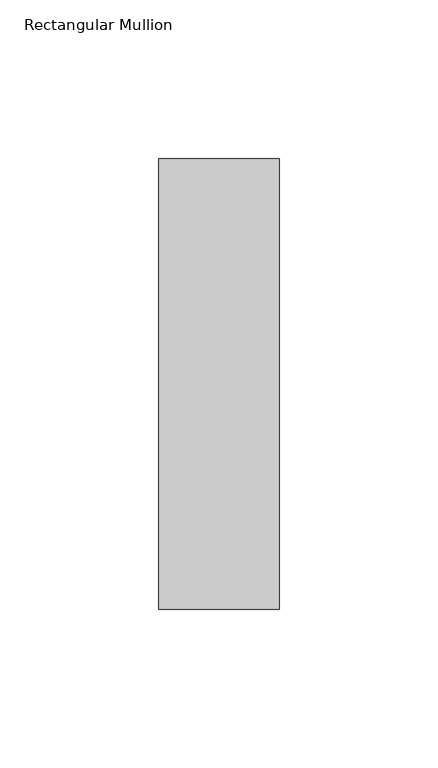
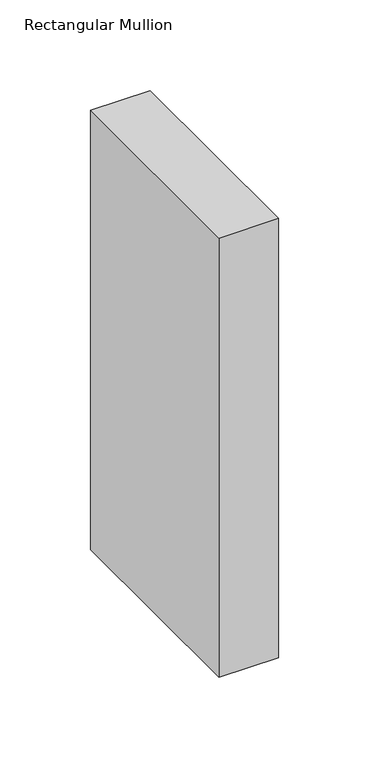
"""IFC4 building model written with IfcOpenShell, lengths in millimetres: member geometry, Rectangular Mullion : NLRS_21_CWM_hsb-regel 38x142_gen_rsf."""

from ifc_helpers import new_model, si_unit, frame, origin, place, context, project, spatial, polyline, outline, extrude, source, transform, mapped, element, save


def rectangular_mullion_567310a4(model_context):
    return source(origin(), model_context, "Body", "SweptSolid", [
        extrude(outline(polyline([(0.0, -71.0), (-38.0, -71.0), (-38.0, 71.0), (0.0, 71.0), (0.0, -71.0)])), frame((0.0, 0.0, -296.0), z_axis=(0.0, 0.0, 1.0), x_axis=(1.0, 0.0, 0.0)), (0.0, 0.0, 1.0), 296.0),
    ])


if __name__ == "__main__":
    model = new_model("IFC4")
    model_context = context("Model", 3, world=origin())
    ifc_project = project(units=[si_unit("LENGTHUNIT", "METRE", prefix="MILLI")], contexts=[model_context])
    site = spatial("IfcSite", under=ifc_project)
    building = spatial("IfcBuilding", under=site)
    placement = place(None, origin())
    rectangular_mullion_shape = rectangular_mullion_567310a4(model_context)
    element("IfcMember", 1, ObjectType="Rectangular Mullion : NLRS_21_CWM_hsb-regel 38x142_gen_rsf", at=placement, inside=building, context=model_context, shape_type="MappedRepresentation", body=[
        mapped(rectangular_mullion_shape, transform((0.0, 0.0, 0.0), x_axis=(1.0, 0.0, 0.0), y_axis=(0.0, 1.0, 0.0), z_axis=(0.0, 0.0, 1.0))),
    ])
    save(model, "model.ifc")

# Revit data of these elements
# Type "Rectangular Mullion : NLRS_21_CWM_hsb-regel 38x142_gen_rsf"
#   Export Type to IFC As = "IfcWall"
#   Type IfcGUID = "07M7mRoiH1CR8m_RSKIwpF"
#   Assembly Code = "21.10"
#   built-in parameter 1007322 = 0.465879 (stored number, unit not read)
#   built-in parameter 1007321 = 0.062336 (stored number, unit not read)
#   built-in parameter 1007320 = 0.062336 (stored number, unit not read)
# Element 1 (IfcMember, "Rectangular Mullion : NLRS_21_CWM_hsb-regel 38x142_gen_rsf")
#   Materials on its faces: "NLRS_i2_hout naaldhout vuren_gen_rsf"
# Materials
#   "NLRS_i2_hout naaldhout vuren_gen_rsf": class "I - Hout", colour RGB 234 199 147, transparency 0, Keynote = "i2", Manufacturer = "Revit Standards Foundation", URL = "www.revitstandards.org", Description = "hout vuren", Cost = 0
